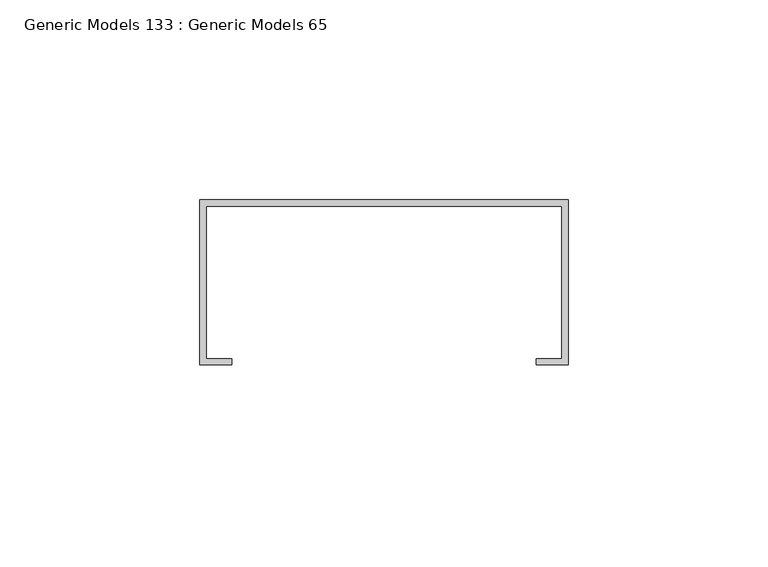
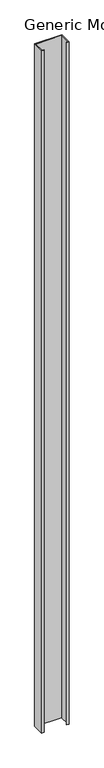
"""IFC4 building model written with IfcOpenShell, lengths in millimetres: proxy geometry, Generic Models 133 : Generic Models 65."""

import ifcopenshell
import ifcopenshell.guid

model = None  # the IFC model being written
_history = None  # IfcOwnerHistory: only IFC2X3 demands one
_inside = {}  # id of a spatial element -> (the spatial element, [elements in it])
_under = {}  # id of a project, library or spatial element -> (it, [spatial elements below it])
_declared = {}  # id of a project -> (the project, [libraries it declares])
_typed = {}  # id of a type object -> (the type object, [elements of that type])
_made_of = {}  # id of a material, layer set ... -> (it, [elements and type objects made of it])


def new_model(schema):
    """Start an empty IFC model of exactly this schema.

    Asked for "IFC4X3", IfcOpenShell would pick the latest addendum, in which some entities
    have other attributes; the version numbers below select the first issue.
    IFC2X3 requires an IfcOwnerHistory on every rooted entity: one is made here for all.
    """
    global model, _history
    if schema == "IFC4X3":
        model = ifcopenshell.file(schema_version=(4, 3, 0, 0))
    else:
        model = ifcopenshell.file(schema=schema)
    _inside.clear()
    _under.clear()
    _declared.clear()
    _typed.clear()
    _made_of.clear()
    _history = None
    if model.schema == "IFC2X3":
        org = make("IfcOrganization", Name="unknown")
        user = make(
            "IfcPersonAndOrganization",
            ThePerson=make("IfcPerson", FamilyName="unknown"),
            TheOrganization=org,
        )
        app = make(
            "IfcApplication",
            ApplicationDeveloper=org,
            Version="unknown",
            ApplicationFullName="unknown",
            ApplicationIdentifier="unknown",
        )
        _history = make(
            "IfcOwnerHistory",
            OwningUser=user,
            OwningApplication=app,
            ChangeAction="ADDED",
            CreationDate=0,
        )
    return model


def make(cls, **values):
    """One entity of the class cls with the attributes given. An attribute that is None is left unset."""
    return model.create_entity(
        cls, **{name: value for name, value in values.items() if value is not None}
    )


def rooted(cls, **values):
    """An entity with a GlobalId (a new one), such as an element, a storey or a relation."""
    return make(cls, GlobalId=ifcopenshell.guid.new(), OwnerHistory=_history, **values)


def si_unit(unit_type, name, prefix=None):
    """IfcSIUnit, for example si_unit("LENGTHUNIT", "METRE", prefix="MILLI")."""
    return make("IfcSIUnit", UnitType=unit_type, Prefix=prefix, Name=name)


def assignment(units):
    """IfcUnitAssignment: the units of a project."""
    return None if units is None else make("IfcUnitAssignment", Units=units)


def point(xyz):
    """IfcCartesianPoint."""
    return None if xyz is None else make("IfcCartesianPoint", Coordinates=xyz)


def direction(xyz):
    """IfcDirection."""
    return None if xyz is None else make("IfcDirection", DirectionRatios=xyz)


def frame(location, z_axis=None, x_axis=None):
    """IfcAxis2Placement3D, a coordinate frame: its origin and axes. An axis left out is left unset."""
    return make(
        "IfcAxis2Placement3D",
        Location=point(location),
        Axis=direction(z_axis),
        RefDirection=direction(x_axis),
    )


def origin():
    """The frame at (0, 0, 0) with its axes left unset."""
    return frame((0.0, 0.0, 0.0))


def place(relative_to, where):
    """IfcLocalPlacement: puts the frame where relative to a parent placement (None: the world)."""
    return make(
        "IfcLocalPlacement", PlacementRelTo=relative_to, RelativePlacement=where
    )


def context(
    kind, dimensions, precision=None, world=None, true_north=None, identifier=None
):
    """IfcGeometricRepresentationContext, for example the 3D "Model" context."""
    return make(
        "IfcGeometricRepresentationContext",
        ContextIdentifier=identifier,
        ContextType=kind,
        CoordinateSpaceDimension=dimensions,
        Precision=precision,
        WorldCoordinateSystem=world,
        TrueNorth=true_north,
    )


def project(units=None, contexts=None):
    """IfcProject with its units and contexts."""
    return rooted(
        "IfcProject",
        Name="project",
        RepresentationContexts=contexts,
        UnitsInContext=assignment(units),
    )


def spatial(cls, under=None, at=None, **own):
    """A site, building, storey or space (cls), placed at a placement, below another one or the project."""
    s = rooted(cls, ObjectPlacement=at, **own)
    if under is not None:
        _under.setdefault(under.id(), (under, []))[1].append(s)
    return s


def polyline(points):
    """IfcPolyline through the points."""
    return make("IfcPolyline", Points=[point(p) for p in points])


def outline(outer, holes=None, kind="AREA"):
    """IfcArbitraryClosedProfileDef: a profile drawn as a closed curve; with holes, ...WithVoids."""
    if holes is None:
        return make("IfcArbitraryClosedProfileDef", ProfileType=kind, OuterCurve=outer)
    return make(
        "IfcArbitraryProfileDefWithVoids",
        ProfileType=kind,
        OuterCurve=outer,
        InnerCurves=holes,
    )


def extrude(swept, where, along, depth):
    """IfcExtrudedAreaSolid: the profile swept, set in the frame where, extruded along a direction by depth."""
    return make(
        "IfcExtrudedAreaSolid",
        SweptArea=swept,
        Position=where,
        ExtrudedDirection=direction(along),
        Depth=depth,
    )


def shape(context_of_items, identifier, shape_type, items):
    """IfcShapeRepresentation: the items that make up one representation, for example the "Body"."""
    return make(
        "IfcShapeRepresentation",
        ContextOfItems=context_of_items,
        RepresentationIdentifier=identifier,
        RepresentationType=shape_type,
        Items=items,
    )


def source(mapping_origin, context_of_items, identifier, shape_type, items):
    """IfcRepresentationMap: a shape defined once, which mapped items show again and again."""
    return make(
        "IfcRepresentationMap",
        MappingOrigin=mapping_origin,
        MappedRepresentation=shape(context_of_items, identifier, shape_type, items),
    )


def transform(
    local_origin,
    x_axis=None,
    y_axis=None,
    z_axis=None,
    scale=None,
    scale2=None,
    scale3=None,
    uniform=True,
):
    """IfcCartesianTransformationOperator3D, or its non-uniform kind. x_axis, y_axis, z_axis: its Axis1, 2, 3."""
    if uniform:
        return make(
            "IfcCartesianTransformationOperator3D",
            Axis1=direction(x_axis),
            Axis2=direction(y_axis),
            LocalOrigin=point(local_origin),
            Scale=scale,
            Axis3=direction(z_axis),
        )
    return make(
        "IfcCartesianTransformationOperator3DnonUniform",
        Axis1=direction(x_axis),
        Axis2=direction(y_axis),
        LocalOrigin=point(local_origin),
        Scale=scale,
        Axis3=direction(z_axis),
        Scale2=scale2,
        Scale3=scale3,
    )


def mapped(mapping_source, mapping_target):
    """IfcMappedItem: shows the shape of a source again, moved by a transform."""
    return make(
        "IfcMappedItem", MappingSource=mapping_source, MappingTarget=mapping_target
    )


def made_of(thing, what):
    """Note that an element or type object is made of a material, layer set ...; save() writes the relation."""
    if what is not None:
        _made_of.setdefault(what.id(), (what, []))[1].append(thing)
    return thing


def element(
    cls,
    number,
    at=None,
    inside=None,
    cuts=None,
    type_object=None,
    material=None,
    context=None,
    identifier="Body",
    shape_type=None,
    held_by="IfcProductDefinitionShape",
    body=None,
    shapes=None,
    **own,
):
    """One element of the class cls, such as IfcWall. Its Tag is "e" and its number.

    at: its placement. inside: the storey or other place that contains it. cuts: it is an
    opening in that element (IfcRelVoidsElement). A single representation is given by context,
    identifier, shape_type and body (its items); several are given by shapes. held_by: the class
    of the entity that holds the representations. save() writes the other relations.
    """
    e = rooted(cls, Tag="e%d" % number, ObjectPlacement=at, **own)
    if body is not None:
        shapes = [shape(context, identifier, shape_type, body)]
    if shapes is not None:
        e.Representation = make(held_by, Representations=shapes)
    if inside is not None:
        _inside.setdefault(inside.id(), (inside, []))[1].append(e)
    if cuts is not None:
        rooted(
            "IfcRelVoidsElement", RelatingBuildingElement=cuts, RelatedOpeningElement=e
        )
    if type_object is not None:
        _typed.setdefault(type_object.id(), (type_object, []))[1].append(e)
    return made_of(e, material)


def aggregate(whole, parts):
    """IfcRelAggregates: a whole, such as a stair, and the parts it consists of."""
    return rooted("IfcRelAggregates", RelatingObject=whole, RelatedObjects=parts)


def save(model, path):
    """Write the relations noted so far, then the file.

    IfcRelAggregates (storeys below a building ...), IfcRelContainedInSpatialStructure (elements
    in a storey), IfcRelDefinesByType, IfcRelAssociatesMaterial and IfcRelDeclares: one each for
    every whole, place, type object, material and project.
    """
    for whole, parts in _under.values():
        aggregate(whole, parts)
    for where, things in _inside.values():
        rooted(
            "IfcRelContainedInSpatialStructure",
            RelatedElements=things,
            RelatingStructure=where,
        )
    for kind, things in _typed.values():
        rooted("IfcRelDefinesByType", RelatedObjects=things, RelatingType=kind)
    for what, things in _made_of.values():
        rooted("IfcRelAssociatesMaterial", RelatedObjects=things, RelatingMaterial=what)
    for by, libraries in _declared.values():
        rooted("IfcRelDeclares", RelatingContext=by, RelatedDefinitions=libraries)
    model.write(path)


def generic_models_133_generic_models_65_9bea1aa1(model_context):
    return source(origin(), model_context, "Body", "SweptSolid", [
        extrude(outline(polyline([(48491.0431639, 630.2375), (48583.1181639, 630.2375), (48583.1181639, 588.9625), (48575.1806639, 588.9625), (48575.1806639, 590.55), (48581.5306639, 590.55), (48581.5306639, 628.65), (48492.6306639, 628.65), (48492.6306639, 590.55), (48498.9806639, 590.55), (48498.9806639, 588.9625), (48491.0431639, 588.9625), (48491.0431639, 630.2375)])), frame((0.0, 0.0, -2148.8358876), z_axis=(0.0, 0.0, 1.0), x_axis=(1.0, 0.0, 0.0)), (0.0, 0.0, 1.0), 2441.575),
    ])


if __name__ == "__main__":
    model = new_model("IFC4")
    model_context = context("Model", 3, world=origin())
    ifc_project = project(units=[si_unit("LENGTHUNIT", "METRE", prefix="MILLI")], contexts=[model_context])
    site = spatial("IfcSite", under=ifc_project)
    building = spatial("IfcBuilding", under=site)
    placement = place(None, origin())
    generic_models_133_generic_models_65_shape = generic_models_133_generic_models_65_9bea1aa1(model_context)
    element("IfcBuildingElementProxy", 1, Name="Generic Models 133 : Generic Models 65", ObjectType="Generic Models 133 : Generic Models 65", at=placement, inside=building, context=model_context, shape_type="MappedRepresentation", body=[
        mapped(generic_models_133_generic_models_65_shape, transform((0.0, 0.0, 0.0), x_axis=(1.0, 0.0, 0.0), y_axis=(0.0, 1.0, 0.0), z_axis=(0.0, 0.0, 1.0))),
    ])
    save(model, "model.ifc")

# Revit data of these elements
# Element 1 (IfcBuildingElementProxy, "Generic Models 133 : Generic Models 65")
#   Materials on its faces: "METAL STUDS - SEE 'WALL TAG' & 'LAYER MATERIAL SCHEDULE' FOR GAUGE/SPACING & INSULATION TREATMENT, IF APPLICABLE"
# Materials
#   "METAL STUDS - SEE 'WALL TAG' & 'LAYER MATERIAL SCHEDULE' FOR GAUGE/SPACING & INSULATION TREATMENT, IF APPLICABLE": class "Unassigned", colour RGB 210 209 208, transparency 0, Keynote = "M05121300.02", Cost = 0
